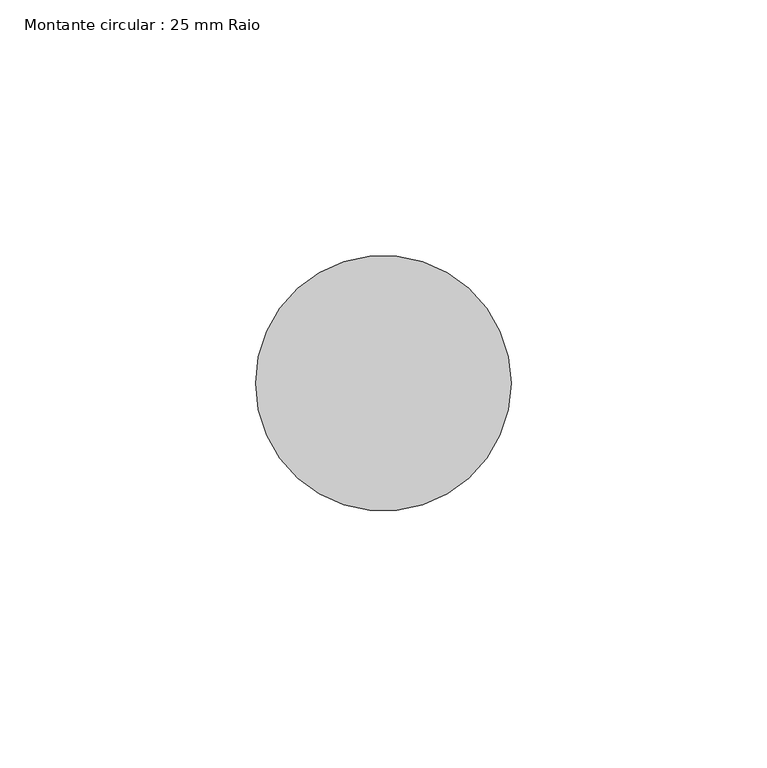
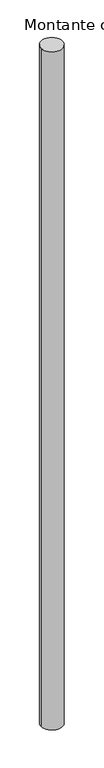
"""IFC4 building model written with IfcOpenShell, lengths in millimetres: member geometry, Montante circular : 25 mm Raio."""

from ifc_helpers import new_model, si_unit, point, frame, origin, origin_2d, place, context, project, spatial, circle_curve, trimmed, segment, composite_curve, outline, extrude, source, transform, mapped, element, save


def montante_circular_25_mm_raio_2f04feea(model_context):
    return source(origin(), model_context, "Body", "SweptSolid", [
        extrude(outline(composite_curve([segment(trimmed(circle_curve(origin_2d(), 25.0), [point((25.0, 0.0))], [point((-25.0, 0.0))], False, "CARTESIAN"), True, "CONTINUOUS"), segment(trimmed(circle_curve(origin_2d(), 25.0), [point((-25.0, 0.0))], [point((25.0, 0.0))], False, "CARTESIAN"), True, "CONTINUOUS")], self_intersect=False)), frame((0.0, 0.0, -1654.9680723), z_axis=(0.0, 0.0, 1.0), x_axis=(1.0, 0.0, 0.0)), (0.0, 0.0, 1.0), 1654.9680723),
    ])


if __name__ == "__main__":
    model = new_model("IFC4")
    model_context = context("Model", 3, world=origin())
    ifc_project = project(units=[si_unit("LENGTHUNIT", "METRE", prefix="MILLI")], contexts=[model_context])
    site = spatial("IfcSite", under=ifc_project)
    building = spatial("IfcBuilding", under=site)
    placement = place(None, origin())
    montante_circular_25_mm_raio_shape = montante_circular_25_mm_raio_2f04feea(model_context)
    element("IfcMember", 1, ObjectType="Montante circular : 25 mm Raio", at=placement, inside=building, context=model_context, shape_type="MappedRepresentation", body=[
        mapped(montante_circular_25_mm_raio_shape, transform((0.0, 0.0, 0.0), x_axis=(1.0, 0.0, 0.0), y_axis=(0.0, 1.0, 0.0), z_axis=(0.0, 0.0, 1.0))),
    ])
    save(model, "model.ifc")

# Revit data of these elements
# Type "Montante circular : 25 mm Raio"
#   built-in parameter 1007350 = 0.082021 (stored number, unit not read)
# Element 1 (IfcMember, "Montante circular : 25 mm Raio")
#   Materials on its faces: "Alumín."
# Materials
#   "Alumín.": class "Metal", colour RGB 247 247 247, transparency 0, Description = "Alumín. 6061", Cost = 0
